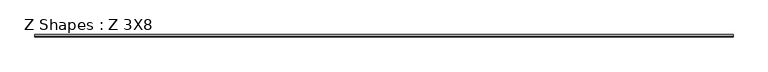
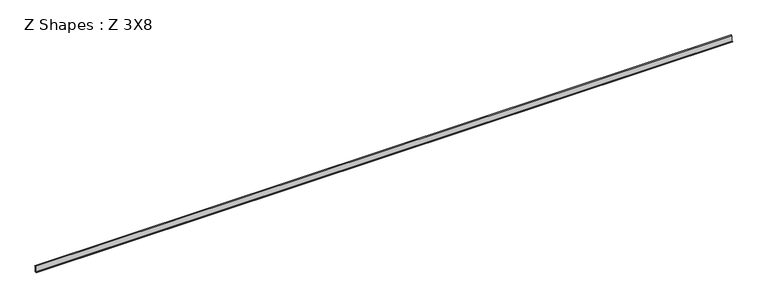
"""IFC4 building model written with IfcOpenShell, lengths in millimetres: beam geometry, Z Shapes : Z 3X8."""

from ifc_helpers import new_model, si_unit, frame, origin, place, context, project, spatial, polyline, outline, extrude, source, transform, mapped, element, save


def z_shapes_z_3x8_f6795473(model_context):
    return source(origin(), model_context, "Body", "SweptSolid", [
        extrude(outline(polyline([(57.2805719, 92.452825), (27.1991352, 92.452825), (27.1991352, -98.809175), (-18.9194281, -98.809175), (-18.9194281, -92.459175), (19.1805719, -92.459175), (19.1805719, 102.104825), (57.2805719, 102.104825), (57.2805719, 92.452825)])), frame((-11474.45, 0.0, 0.0), z_axis=(1.0, 0.0, 0.0), x_axis=(0.0, 1.0, 0.0)), (0.0, 0.0, 1.0), 23361.65),
    ])


if __name__ == "__main__":
    model = new_model("IFC4")
    model_context = context("Model", 3, world=origin())
    ifc_project = project(units=[si_unit("LENGTHUNIT", "METRE", prefix="MILLI")], contexts=[model_context])
    site = spatial("IfcSite", under=ifc_project)
    building = spatial("IfcBuilding", under=site)
    placement = place(None, origin())
    z_shapes_z_3x8_shape = z_shapes_z_3x8_f6795473(model_context)
    element("IfcBeam", 1, ObjectType="Z Shapes : Z 3X8", at=placement, inside=building, context=model_context, shape_type="MappedRepresentation", body=[
        mapped(z_shapes_z_3x8_shape, transform((0.0, 0.0, 0.0), x_axis=(1.0, 0.0, 0.0), y_axis=(0.0, 1.0, 0.0), z_axis=(0.0, 0.0, 1.0))),
    ])
    save(model, "model.ifc")

# Revit data of these elements
# Type "Z Shapes : Z 3X8"
#   Section Name Key = "W12x26"
#   Assembly Code = "B10"
#   Width = 76.2 mm
#   Web Thickness = 5.842 mm
#   Web Fillet = 7.62 mm
#   Warping Constant = 163001.3 cm⁶
#   Torsional Moment of Inertia = 12.4869 cm⁴
#   Section Area = 7.65 in²
#   Plastic Modulus weak axis = 0.00472801 (stored number, unit not read)
#   Plastic Modulus strong axis = 0.0215278 (stored number, unit not read)
#   Perimeter = 15.0571 m²/m
#   Nominal Weight = 379.441 N/m
#   Moment of Inertia weak axis = 720.08 cm⁴
#   Moment of Inertia strong axis = 8491.12 cm⁴
#   Height = 184.912 mm
#   Flange Thickness = 9.652 mm
#   Elastic Modulus weak axis = 0.00309028 (stored number, unit not read)
#   Elastic Modulus strong axis = 0.0193287 (stored number, unit not read)
#   Centroid Vertical = 92.456 mm
#   Centroid Horizontal = 38.1 mm
#   Length [instance default] = 5' - 0"
#   Structural Material [instance default] = Steel ASTM A992
#   Principal Axes Angle = 0
# Element 1 (IfcBeam, "Z Shapes : Z 3X8")
#   Materials on its faces: "Steel ASTM A992"
# Materials
#   "Steel ASTM A992": class "Metal", colour RGB 189 187 185, transparency 0, Description = "Structural steel 50ksi", Cost = 0
